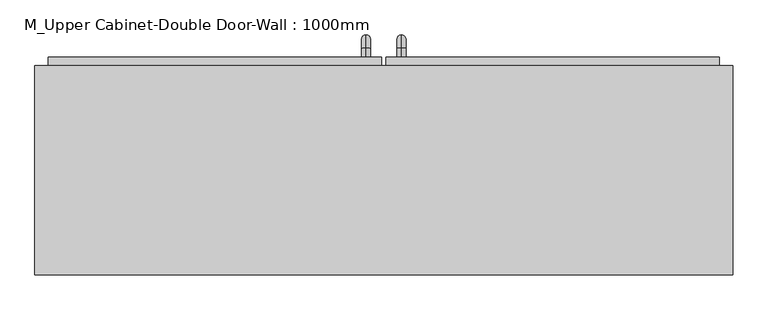
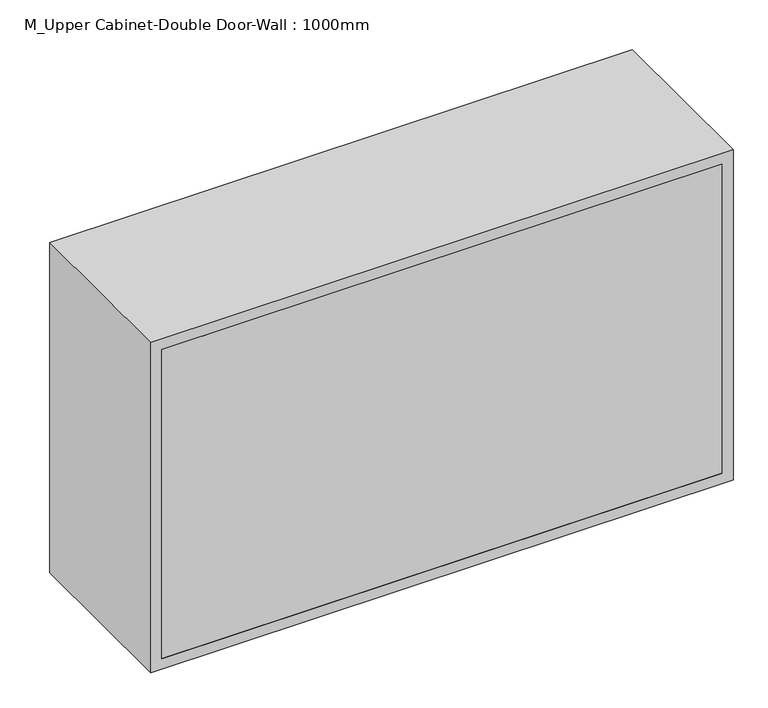
"""IFC4 building model written with IfcOpenShell, lengths in millimetres: furniture geometry, M_Upper Cabinet-Double Door-Wall : 1000mm."""

from ifc_helpers import new_model, si_unit, point, frame, origin, place, context, project, spatial, polyline, circle_curve, ellipse_curve, trimmed, outline, extrude, source, transform, mapped, element, save
from ifc_brep_helpers import plane_surface, cylinder_surface, revolved_surface, advanced_brep


def m_upper_cabinet_double_door_wall_1000mm_05d7b990(model_context):
    return source(origin(), model_context, "Body", "SolidModel", [
        extrude(outline(polyline([(2000.0, -470.2288372), (1400.0, -470.2288372), (1400.0, 529.7711628), (2000.0, 529.7711628), (2000.0, -470.2288372)]), holes=[polyline([(1980.95, -451.1788372), (1980.95, 510.7211628), (1419.05, 510.7211628), (1419.05, -451.1788372), (1980.95, -451.1788372)])]), frame((0.0, 62.5, 0.0), z_axis=(0.0, 1.0, 0.0), x_axis=(0.0, 0.0, 1.0)), (0.0, 0.0, 1.0), 300.0),
        extrude(outline(polyline([(510.7211628, 62.5), (-451.1788372, 62.5), (-451.1788372, 81.55), (510.7211628, 81.55), (510.7211628, 62.5)])), frame((0.0, 0.0, 1419.05), z_axis=(0.0, 0.0, 1.0), x_axis=(1.0, 0.0, 0.0)), (0.0, 0.0, 1.0), 561.9),
        extrude(outline(polyline([(32.9461628, 375.2), (510.7211628, 375.2), (510.7211628, 343.45), (32.9461628, 343.45), (32.9461628, 375.2)])), frame((0.0, 0.0, 1419.05), z_axis=(0.0, 0.0, 1.0), x_axis=(1.0, 0.0, 0.0)), (0.0, 0.0, 1.0), 561.9),
        extrude(outline(polyline([(-451.1788372, 375.2), (26.5961628, 375.2), (26.5961628, 343.45), (-451.1788372, 343.45), (-451.1788372, 375.2)])), frame((0.0, 0.0, 1419.05), z_axis=(0.0, 0.0, 1.0), x_axis=(1.0, 0.0, 0.0)), (0.0, 0.0, 1.0), 561.9),
        advanced_brep(
        [(4.3711628, 375.2, 1546.05), (4.3711628, 375.2, 1558.75), (4.3711628, 387.9, 1546.05), (4.3711628, 387.9, 1558.75), (4.3711628, 406.95, 1539.7), (4.3711628, 394.25, 1539.7), (4.3711628, 394.25, 1463.5), (4.3711628, 406.95, 1463.5), (4.3711628, 387.9, 1444.45), (4.3711628, 387.9, 1457.15), (4.3711628, 375.2, 1457.15), (4.3711628, 375.2, 1444.45)],
        [
            (0, 1, circle_curve(frame((4.3711628, 375.2, 1552.4), z_axis=(0.0, -1.0, 0.0), x_axis=(0.0, 0.0, 1.0)), 6.35)),
            (1, 0, circle_curve(frame((4.3711628, 375.2, 1552.4), z_axis=(0.0, -1.0, 0.0), x_axis=(0.0, 0.0, 1.0)), 6.35)),
            (0, 2),
            (2, 3, circle_curve(frame((4.3711628, 387.9, 1552.4), z_axis=(0.0, -1.0, 0.0), x_axis=(0.0, 0.0, 1.0)), 6.35)),
            (3, 1),
            (3, 2, circle_curve(frame((4.3711628, 387.9, 1552.4), z_axis=(0.0, -1.0, 0.0), x_axis=(0.0, 0.0, 1.0)), 6.35)),
            (4, 3, circle_curve(frame((4.3711628, 387.9, 1539.7), z_axis=(1.0, 0.0, 0.0), x_axis=(0.0, 0.0, 1.0)), 19.05)),
            (2, 5, circle_curve(frame((4.3711628, 387.9, 1539.7), z_axis=(-1.0, 0.0, 0.0), x_axis=(0.0, 0.0, 1.0)), 6.35)),
            (5, 4, circle_curve(frame((4.3711628, 400.6, 1539.7), z_axis=(0.0, 0.0, 1.0), x_axis=(0.0, 1.0, 0.0)), 6.35)),
            (4, 5, circle_curve(frame((4.3711628, 400.6, 1539.7), z_axis=(0.0, 0.0, 1.0), x_axis=(0.0, 1.0, 0.0)), 6.35)),
            (5, 6),
            (6, 7, circle_curve(frame((4.3711628, 400.6, 1463.5), z_axis=(0.0, 0.0, 1.0), x_axis=(0.0, 1.0, 0.0)), 6.35)),
            (7, 4),
            (7, 6, circle_curve(frame((4.3711628, 400.6, 1463.5), z_axis=(0.0, 0.0, 1.0), x_axis=(0.0, 1.0, 0.0)), 6.35)),
            (8, 7, circle_curve(frame((4.3711628, 387.9, 1463.5), z_axis=(1.0, 0.0, 0.0), x_axis=(0.0, 1.0, 0.0)), 19.05)),
            (6, 9, circle_curve(frame((4.3711628, 387.9, 1463.5), z_axis=(-1.0, 0.0, 0.0), x_axis=(0.0, 1.0, 0.0)), 6.35)),
            (9, 8, circle_curve(frame((4.3711628, 387.9, 1450.8), z_axis=(0.0, 1.0, 0.0), x_axis=(0.0, 0.0, -1.0)), 6.35)),
            (8, 9, circle_curve(frame((4.3711628, 387.9, 1450.8), z_axis=(0.0, 1.0, 0.0), x_axis=(0.0, 0.0, -1.0)), 6.35)),
            (10, 11, circle_curve(frame((4.3711628, 375.2, 1450.8), z_axis=(0.0, -1.0, 0.0), x_axis=(0.0, 0.0, -1.0)), 6.35)),
            (11, 10, circle_curve(frame((4.3711628, 375.2, 1450.8), z_axis=(0.0, -1.0, 0.0), x_axis=(0.0, 0.0, -1.0)), 6.35)),
            (9, 10),
            (11, 8),
        ],
        [
            plane_surface(frame((-1.9788372, 375.2, 1552.4), z_axis=(0.0, -1.0, 0.0), x_axis=(0.0, 0.0, 1.0))),
            cylinder_surface(frame((4.3711628, 375.2, 1552.4), z_axis=(0.0, -1.0, 0.0), x_axis=(0.0, 0.0, 1.0)), 6.35),
            revolved_surface(trimmed(ellipse_curve(frame((4.3711628, 387.9, 1552.4), z_axis=(0.0, -1.0, 0.0), x_axis=(0.0, 0.0, 1.0)), 6.35, 6.35), [point((4.3711628, 387.9, 1546.05))], [point((4.3711628, 387.9, 1558.75))], True, "CARTESIAN"), (4.3711628, 387.9, 1539.7), (-1.0, 0.0, 0.0)),
            revolved_surface(trimmed(ellipse_curve(frame((4.3711628, 387.9, 1552.4), z_axis=(0.0, -1.0, 0.0), x_axis=(0.0, 0.0, 1.0)), 6.35, 6.35), [point((4.3711628, 387.9, 1558.75))], [point((4.3711628, 387.9, 1546.05))], True, "CARTESIAN"), (4.3711628, 387.9, 1539.7), (-1.0, 0.0, 0.0)),
            cylinder_surface(frame((4.3711628, 400.6, 1539.7), z_axis=(0.0, 0.0, 1.0), x_axis=(0.0, 1.0, 0.0)), 6.35),
            revolved_surface(trimmed(ellipse_curve(frame((4.3711628, 400.6, 1463.5), z_axis=(0.0, 0.0, 1.0), x_axis=(0.0, 1.0, 0.0)), 6.35, 6.35), [point((4.3711628, 394.25, 1463.5))], [point((4.3711628, 406.95, 1463.5))], True, "CARTESIAN"), (4.3711628, 387.9, 1463.5), (-1.0, 0.0, 0.0)),
            revolved_surface(trimmed(ellipse_curve(frame((4.3711628, 400.6, 1463.5), z_axis=(0.0, 0.0, 1.0), x_axis=(0.0, 1.0, 0.0)), 6.35, 6.35), [point((4.3711628, 406.95, 1463.5))], [point((4.3711628, 394.25, 1463.5))], True, "CARTESIAN"), (4.3711628, 387.9, 1463.5), (-1.0, 0.0, 0.0)),
            plane_surface(frame((-1.9788372, 375.2, 1450.8), z_axis=(0.0, -1.0, 0.0), x_axis=(0.0, 0.0, -1.0))),
            cylinder_surface(frame((4.3711628, 387.9, 1450.8), z_axis=(0.0, 1.0, 0.0), x_axis=(0.0, 0.0, -1.0)), 6.35),
        ],
        [
            (0, [[1, 2]]),
            (1, [[-1, 3, 4, 5]]),
            (1, [[-2, -5, 6, -3]]),
            (2, [[7, -4, 8, 9]]),
            (3, [[-8, -6, -7, 10]]),
            (4, [[-9, 11, 12, 13]]),
            (4, [[-10, -13, 14, -11]]),
            (5, [[15, -12, 16, 17]]),
            (6, [[-16, -14, -15, 18]]),
            (7, [[19, 20]]),
            (8, [[-17, 21, -20, 22]]),
            (8, [[-18, -22, -19, -21]]),
        ],
    ),
        advanced_brep(
        [(55.1711628, 375.2, 1546.05), (55.1711628, 375.2, 1558.75), (55.1711628, 387.9, 1546.05), (55.1711628, 387.9, 1558.75), (55.1711628, 406.95, 1539.7), (55.1711628, 394.25, 1539.7), (55.1711628, 394.25, 1463.5), (55.1711628, 406.95, 1463.5), (55.1711628, 387.9, 1444.45), (55.1711628, 387.9, 1457.15), (55.1711628, 375.2, 1457.15), (55.1711628, 375.2, 1444.45)],
        [
            (0, 1, circle_curve(frame((55.1711628, 375.2, 1552.4), z_axis=(0.0, -1.0, 0.0), x_axis=(0.0, 0.0, -1.0)), 6.35)),
            (1, 0, circle_curve(frame((55.1711628, 375.2, 1552.4), z_axis=(0.0, -1.0, 0.0), x_axis=(0.0, 0.0, -1.0)), 6.35)),
            (0, 2),
            (2, 3, circle_curve(frame((55.1711628, 387.9, 1552.4), z_axis=(0.0, -1.0, 0.0), x_axis=(0.0, 0.0, -1.0)), 6.35)),
            (3, 1),
            (3, 2, circle_curve(frame((55.1711628, 387.9, 1552.4), z_axis=(0.0, -1.0, 0.0), x_axis=(0.0, 0.0, -1.0)), 6.35)),
            (4, 3, circle_curve(frame((55.1711628, 387.9, 1539.7), z_axis=(1.0, 0.0, 0.0), x_axis=(0.0, 0.0, 1.0)), 19.05)),
            (2, 5, circle_curve(frame((55.1711628, 387.9, 1539.7), z_axis=(-1.0, 0.0, 0.0), x_axis=(0.0, 0.0, 1.0)), 6.35)),
            (5, 4, circle_curve(frame((55.1711628, 400.6, 1539.7), z_axis=(0.0, 0.0, 1.0), x_axis=(0.0, -1.0, 0.0)), 6.35)),
            (4, 5, circle_curve(frame((55.1711628, 400.6, 1539.7), z_axis=(0.0, 0.0, 1.0), x_axis=(0.0, -1.0, 0.0)), 6.35)),
            (5, 6),
            (6, 7, circle_curve(frame((55.1711628, 400.6, 1463.5), z_axis=(0.0, 0.0, 1.0), x_axis=(0.0, -1.0, 0.0)), 6.35)),
            (7, 4),
            (7, 6, circle_curve(frame((55.1711628, 400.6, 1463.5), z_axis=(0.0, 0.0, 1.0), x_axis=(0.0, -1.0, 0.0)), 6.35)),
            (8, 7, circle_curve(frame((55.1711628, 387.9, 1463.5), z_axis=(1.0, 0.0, 0.0), x_axis=(0.0, 1.0, 0.0)), 19.05)),
            (6, 9, circle_curve(frame((55.1711628, 387.9, 1463.5), z_axis=(-1.0, 0.0, 0.0), x_axis=(0.0, 1.0, 0.0)), 6.35)),
            (9, 8, circle_curve(frame((55.1711628, 387.9, 1450.8), z_axis=(0.0, 1.0, 0.0), x_axis=(0.0, 0.0, 1.0)), 6.35)),
            (8, 9, circle_curve(frame((55.1711628, 387.9, 1450.8), z_axis=(0.0, 1.0, 0.0), x_axis=(0.0, 0.0, 1.0)), 6.35)),
            (10, 11, circle_curve(frame((55.1711628, 375.2, 1450.8), z_axis=(0.0, -1.0, 0.0), x_axis=(0.0, 0.0, 1.0)), 6.35)),
            (11, 10, circle_curve(frame((55.1711628, 375.2, 1450.8), z_axis=(0.0, -1.0, 0.0), x_axis=(0.0, 0.0, 1.0)), 6.35)),
            (9, 10),
            (11, 8),
        ],
        [
            plane_surface(frame((48.8211628, 375.2, 1552.4), z_axis=(0.0, -1.0, 0.0), x_axis=(0.0, 0.0, 1.0))),
            cylinder_surface(frame((55.1711628, 375.2, 1552.4), z_axis=(0.0, -1.0, 0.0), x_axis=(0.0, 0.0, -1.0)), 6.35),
            revolved_surface(trimmed(ellipse_curve(frame((55.1711628, 387.9, 1552.4), z_axis=(0.0, -1.0, 0.0), x_axis=(0.0, 0.0, -1.0)), 6.35, 6.35), [point((55.1711628, 387.9, 1546.05))], [point((55.1711628, 387.9, 1558.75))], True, "CARTESIAN"), (55.1711628, 387.9, 1539.7), (-1.0, 0.0, 0.0)),
            revolved_surface(trimmed(ellipse_curve(frame((55.1711628, 387.9, 1552.4), z_axis=(0.0, -1.0, 0.0), x_axis=(0.0, 0.0, -1.0)), 6.35, 6.35), [point((55.1711628, 387.9, 1558.75))], [point((55.1711628, 387.9, 1546.05))], True, "CARTESIAN"), (55.1711628, 387.9, 1539.7), (-1.0, 0.0, 0.0)),
            cylinder_surface(frame((55.1711628, 400.6, 1539.7), z_axis=(0.0, 0.0, 1.0), x_axis=(0.0, -1.0, 0.0)), 6.35),
            revolved_surface(trimmed(ellipse_curve(frame((55.1711628, 400.6, 1463.5), z_axis=(0.0, 0.0, 1.0), x_axis=(0.0, -1.0, 0.0)), 6.35, 6.35), [point((55.1711628, 394.25, 1463.5))], [point((55.1711628, 406.95, 1463.5))], True, "CARTESIAN"), (55.1711628, 387.9, 1463.5), (-1.0, 0.0, 0.0)),
            revolved_surface(trimmed(ellipse_curve(frame((55.1711628, 400.6, 1463.5), z_axis=(0.0, 0.0, 1.0), x_axis=(0.0, -1.0, 0.0)), 6.35, 6.35), [point((55.1711628, 406.95, 1463.5))], [point((55.1711628, 394.25, 1463.5))], True, "CARTESIAN"), (55.1711628, 387.9, 1463.5), (-1.0, 0.0, 0.0)),
            plane_surface(frame((48.8211628, 375.2, 1450.8), z_axis=(0.0, -1.0, 0.0), x_axis=(0.0, 0.0, -1.0))),
            cylinder_surface(frame((55.1711628, 387.9, 1450.8), z_axis=(0.0, 1.0, 0.0), x_axis=(0.0, 0.0, 1.0)), 6.35),
        ],
        [
            (0, [[1, 2]]),
            (1, [[-1, 3, 4, 5]]),
            (1, [[-2, -5, 6, -3]]),
            (2, [[7, -4, 8, 9]]),
            (3, [[-8, -6, -7, 10]]),
            (4, [[-9, 11, 12, 13]]),
            (4, [[-10, -13, 14, -11]]),
            (5, [[15, -12, 16, 17]]),
            (6, [[-16, -14, -15, 18]]),
            (7, [[19, 20]]),
            (8, [[-17, 21, -20, 22]]),
            (8, [[-18, -22, -19, -21]]),
        ],
    ),
    ])


if __name__ == "__main__":
    model = new_model("IFC4")
    model_context = context("Model", 3, world=origin())
    ifc_project = project(units=[si_unit("LENGTHUNIT", "METRE", prefix="MILLI")], contexts=[model_context])
    site = spatial("IfcSite", under=ifc_project)
    building = spatial("IfcBuilding", under=site)
    placement = place(None, origin())
    m_upper_cabinet_double_door_wall_1000mm_shape = m_upper_cabinet_double_door_wall_1000mm_05d7b990(model_context)
    element("IfcFurniture", 1, ObjectType="M_Upper Cabinet-Double Door-Wall : 1000mm", at=placement, inside=building, context=model_context, shape_type="MappedRepresentation", body=[
        mapped(m_upper_cabinet_double_door_wall_1000mm_shape, transform((0.0, 0.0, 0.0), x_axis=(1.0, 0.0, 0.0), y_axis=(0.0, 1.0, 0.0), z_axis=(0.0, 0.0, 1.0))),
    ])
    save(model, "model.ifc")

# Revit data of these elements
# Type "M_Upper Cabinet-Double Door-Wall : 1000mm"
#   Depth = 300 mm
#   Height = 600 mm
#   Top Of Cabinet = 2000 mm
#   Width = 1000 mm
#   Cabinet Material = none
#   Door/Drawer Material = none
#   Handle Material = Cabinets - Handles
#   Default Elevation = 0
# Element 1 (IfcFurniture, "M_Upper Cabinet-Double Door-Wall : 1000mm")
#   Materials on its faces: "Cabinets", "Cabinets - Handles"
# Materials
#   "Cabinets - Handles": class "Metal", colour RGB 57 57 57, transparency 0, Cost = 0
#   "Cabinets": class "Miscellaneous", colour RGB 249 249 249, transparency 0, Cost = 0
